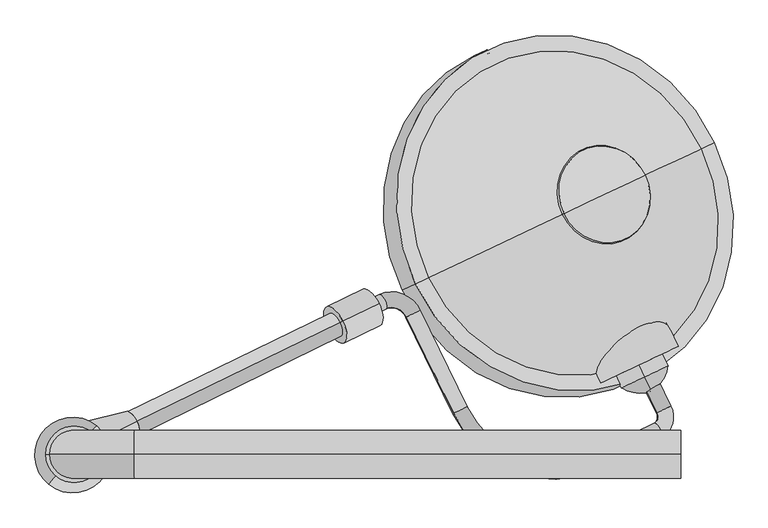
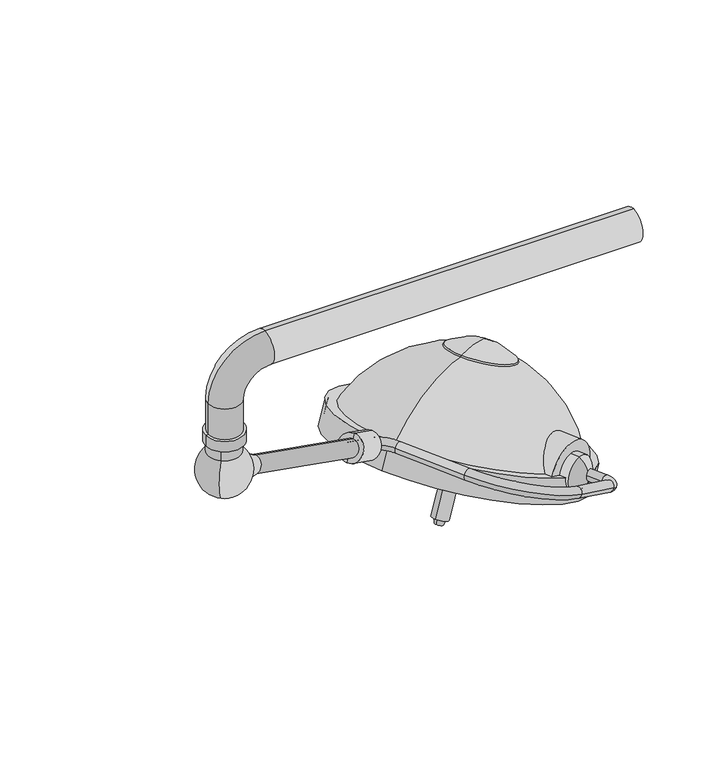
"""IFC4 building model written with IfcOpenShell, lengths in millimetres: proxy geometry, M7485 - Light, Surg, Ceiling Mtd, Dual, Equal Dia Heads : M7485 - Light, Surg, Ceiling Mtd, Dual, Equal Dia Heads."""

from ifc_helpers import new_model, si_unit, point, frame, frame_2d, origin, origin_2d, place, context, project, spatial, polyline, circle_curve, ellipse_curve, trimmed, segment, composite_curve, outline, extrude, source, transform, mapped, element, save
from ifc_brep_helpers import plane_surface, cylinder_surface, revolved_surface, advanced_brep


def specialty_equipment_14047777(model_context):
    return source(origin(), model_context, "Body", "SolidModel", [
        advanced_brep(
        [(-51.3241797, -670.2413617, 1699.7604265), (-72.1798458, -680.4133498, 1710.0915373), (-51.503984, -722.8051486, 1710.0915373), (-30.6483179, -712.6331606, 1699.7604265), (-56.3645035, -739.305827, 1715.2570926), (-45.2298764, -762.1351958, 1715.2570926), (-159.8794514, -789.7934405, 1766.5344952), (-148.7448243, -812.6228093, 1766.5344952), (-351.8212111, -713.8491561, 1828.5211596), (-372.6768772, -724.0211441, 1838.8522704), (-426.0821694, -561.5916279, 1828.5211596), (-446.9378356, -571.7636159, 1838.8522704), (-490.062756, -536.2768664, 1849.1833811), (-478.9281288, -559.1062352, 1849.1833811), (-557.8921303, -597.619552, 1888.2991704), (-569.0267574, -574.7901832, 1888.2991704)],
        [
            (0, 1, circle_curve(frame((-61.7520127, -675.3273558, 1704.9259819), z_axis=(-0.43837114678908723, 0.8987940462991623, 0.0), x_axis=(-0.8210892183528129, -0.40047196991074896, 0.4067366430758003)), 12.7)),
            (1, 0, circle_curve(frame((-61.7520127, -675.3273558, 1704.9259819), z_axis=(-0.43837114678908723, 0.8987940462991623, 0.0), x_axis=(-0.8210892183528129, -0.40047196991074896, 0.4067366430758003)), 12.7)),
            (1, 2),
            (2, 3, circle_curve(frame((-41.0761509, -717.7191546, 1704.9259819), z_axis=(-0.43837114678908723, 0.8987940462991623, 0.0), x_axis=(-0.8210892183528129, -0.40047196991074896, 0.4067366430758003)), 12.7)),
            (3, 0),
            (3, 2, circle_curve(frame((-41.0761509, -717.7191546, 1704.9259819), z_axis=(-0.43837114678908723, 0.8987940462991623, 0.0), x_axis=(-0.8210892183528129, -0.40047196991074896, 0.4067366430758003)), 12.7)),
            (4, 5, circle_curve(frame((-50.79719, -750.7205114, 1715.2570926), z_axis=(0.8210892183528035, 0.4004719699107681, -0.4067366430758003), x_axis=(-0.43837114678910477, 0.8987940462991536, 0.0)), 12.7)),
            (5, 3, circle_curve(frame((-61.9318171, -727.8911427, 1715.2570926), z_axis=(0.36557247320823727, 0.17830160866628114, 0.9135454576426009), x_axis=(0.8210892183528128, 0.400471969910749, -0.4067366430758004)), 38.1)),
            (2, 4, circle_curve(frame((-61.9318171, -727.8911427, 1715.2570926), z_axis=(-0.36557247320823727, -0.17830160866628114, -0.9135454576426009), x_axis=(0.8210892183528128, 0.400471969910749, -0.4067366430758004)), 12.7)),
            (5, 4, circle_curve(frame((-50.79719, -750.7205114, 1715.2570926), z_axis=(0.8210892183528112, 0.4004719699107522, -0.4067366430758003), x_axis=(-0.4383711467890902, 0.8987940462991607, 0.0)), 12.7)),
            (4, 6),
            (6, 7, circle_curve(frame((-154.3121378, -801.2081249, 1766.5344952), z_axis=(0.821089218352813, 0.40047196991074857, -0.40673664307580043), x_axis=(-0.4383711467890869, 0.8987940462991624, 0.0)), 12.7)),
            (7, 5),
            (7, 6, circle_curve(frame((-154.3121378, -801.2081249, 1766.5344952), z_axis=(0.821089218352813, 0.40047196991074857, -0.40673664307580043), x_axis=(-0.4383711467890869, 0.8987940462991624, 0.0)), 12.7)),
            (8, 9, circle_curve(frame((-362.2490441, -718.9351501, 1833.686715), z_axis=(0.4383711467890848, -0.8987940462991635, 0.0), x_axis=(0.8210892183528142, 0.4004719699107463, -0.40673664307580043)), 12.7)),
            (9, 7, circle_curve(frame((-226.6872142, -652.8172279, 1766.5344952), z_axis=(0.36557247320823727, 0.17830160866628114, 0.9135454576426009), x_axis=(0.43837114678909317, -0.8987940462991594, 0.0)), 177.8)),
            (6, 8, circle_curve(frame((-226.6872142, -652.8172279, 1766.5344952), z_axis=(-0.36557247320823727, -0.17830160866628114, -0.9135454576426009), x_axis=(0.43837114678909317, -0.8987940462991594, 0.0)), 152.4)),
            (9, 8, circle_curve(frame((-362.2490441, -718.9351501, 1833.686715), z_axis=(0.4383711467890851, -0.8987940462991633, 0.0), x_axis=(0.821089218352814, 0.40047196991074674, -0.40673664307580043)), 12.7)),
            (8, 10),
            (10, 11, circle_curve(frame((-436.5100025, -566.6776219, 1833.686715), z_axis=(0.43837114678908545, -0.898794046299163, 0.0), x_axis=(0.8210892183528139, 0.400471969910747, -0.4067366430758005)), 12.7)),
            (11, 9),
            (11, 10, circle_curve(frame((-436.5100025, -566.6776219, 1833.686715), z_axis=(0.43837114678908545, -0.898794046299163, 0.0), x_axis=(0.8210892183528139, 0.400471969910747, -0.4067366430758005)), 12.7)),
            (12, 13, circle_curve(frame((-484.4954424, -547.6915508, 1849.1833811), z_axis=(0.8210892183528171, 0.40047196991074047, -0.4067366430758004), x_axis=(-0.4383711467890795, 0.898794046299166, 0.0)), 12.7)),
            (13, 11, circle_curve(frame((-467.7935017, -581.935604, 1849.1833811), z_axis=(-0.36557247320823727, -0.17830160866628114, -0.9135454576426009), x_axis=(0.8210892183528169, 0.4004719699107408, -0.4067366430758004)), 25.4)),
            (10, 12, circle_curve(frame((-467.7935017, -581.935604, 1849.1833811), z_axis=(0.36557247320823727, 0.17830160866628114, 0.9135454576426009), x_axis=(0.8210892183528169, 0.4004719699107408, -0.4067366430758004)), 50.8)),
            (13, 12, circle_curve(frame((-484.4954424, -547.6915508, 1849.1833811), z_axis=(0.8210892183528171, 0.40047196991074047, -0.4067366430758004), x_axis=(-0.4383711467890795, 0.898794046299166, 0.0)), 12.7)),
            (14, 15, circle_curve(frame((-563.4594439, -586.2048676, 1888.2991704), z_axis=(-0.821089218352815, -0.40047196991074563, 0.4067366430757997), x_axis=(-0.438371146789084, 0.8987940462991637, 0.0)), 12.7)),
            (15, 14, circle_curve(frame((-563.4594439, -586.2048676, 1888.2991704), z_axis=(-0.821089218352815, -0.40047196991074563, 0.4067366430757997), x_axis=(-0.438371146789084, 0.8987940462991637, 0.0)), 12.7)),
            (12, 15),
            (14, 13),
        ],
        [
            plane_surface(frame((-671.2712366, -972.6097446, 181.7710423), z_axis=(-0.43837114678908734, 0.8987940462991622, 0.0), x_axis=(0.3655724732082375, 0.17830160866628114, 0.9135454576426008))),
            cylinder_surface(frame((-61.7520127, -675.3273558, 1704.9259819), z_axis=(-0.43837114678908723, 0.8987940462991623, 0.0), x_axis=(-0.8210892183528129, -0.40047196991074896, 0.4067366430758003)), 12.7),
            revolved_surface(trimmed(ellipse_curve(frame((-41.0761509, -717.7191546, 1704.9259819), z_axis=(0.43837114678908723, -0.8987940462991622, 0.0), x_axis=(-0.8210892183528128, -0.4004719699107489, 0.40673664307580043)), 12.7, 12.7), [point((-30.6483179, -712.6331606, 1699.7604265))], [point((-51.503984, -722.8051486, 1710.0915373))], True, "CARTESIAN"), (-671.451041, -1025.1735315, 192.1021531), (0.36557247320823727, 0.17830160866628114, 0.9135454576426009)),
            revolved_surface(trimmed(ellipse_curve(frame((-41.0761509, -717.7191546, 1704.9259819), z_axis=(0.43837114678908723, -0.8987940462991622, 0.0), x_axis=(-0.8210892183528128, -0.4004719699107489, 0.40673664307580043)), 12.7, 12.7), [point((-51.503984, -722.8051486, 1710.0915373))], [point((-30.6483179, -712.6331606, 1699.7604265))], True, "CARTESIAN"), (-671.451041, -1025.1735315, 192.1021531), (0.36557247320823727, 0.17830160866628114, 0.9135454576426009)),
            cylinder_surface(frame((-50.79719, -750.7205114, 1715.2570926), z_axis=(0.821089218352813, 0.40047196991074857, -0.40673664307580043), x_axis=(-0.4383711467890869, 0.8987940462991624, 0.0)), 12.7),
            revolved_surface(trimmed(ellipse_curve(frame((-154.3121378, -801.2081249, 1766.5344952), z_axis=(-0.8210892183528098, -0.40047196991075545, 0.4067366430758005), x_axis=(-0.4383711467890932, 0.8987940462991594, 0.0)), 12.7, 12.7), [point((-148.7448243, -812.6228093, 1766.5344952))], [point((-159.8794514, -789.7934405, 1766.5344952))], True, "CARTESIAN"), (-836.2064381, -950.0996167, 243.3795556), (0.36557247320823727, 0.17830160866628114, 0.9135454576426009)),
            revolved_surface(trimmed(ellipse_curve(frame((-154.3121378, -801.2081249, 1766.5344952), z_axis=(-0.8210892183528098, -0.40047196991075545, 0.4067366430758005), x_axis=(-0.4383711467890932, 0.8987940462991594, 0.0)), 12.7, 12.7), [point((-159.8794514, -789.7934405, 1766.5344952))], [point((-148.7448243, -812.6228093, 1766.5344952))], True, "CARTESIAN"), (-836.2064381, -950.0996167, 243.3795556), (0.36557247320823727, 0.17830160866628114, 0.9135454576426009)),
            cylinder_surface(frame((-362.2490441, -718.9351501, 1833.686715), z_axis=(0.43837114678908556, -0.8987940462991633, 0.0), x_axis=(0.8210892183528139, 0.400471969910747, -0.4067366430758005)), 12.7),
            revolved_surface(trimmed(ellipse_curve(frame((-436.5100025, -566.6776219, 1833.686715), z_axis=(-0.43837114678907957, 0.898794046299166, 0.0), x_axis=(0.821089218352817, 0.4004719699107405, -0.40673664307580043)), 12.7, 12.7), [point((-446.9378356, -571.7636159, 1838.8522704))], [point((-426.0821694, -561.5916279, 1828.5211596))], True, "CARTESIAN"), (-1077.3127256, -879.2179928, 326.0284415), (-0.36557247320823727, -0.17830160866628114, -0.9135454576426009)),
            revolved_surface(trimmed(ellipse_curve(frame((-436.5100025, -566.6776219, 1833.686715), z_axis=(-0.43837114678907957, 0.898794046299166, 0.0), x_axis=(0.821089218352817, 0.4004719699107405, -0.40673664307580043)), 12.7, 12.7), [point((-426.0821694, -561.5916279, 1828.5211596))], [point((-446.9378356, -571.7636159, 1838.8522704))], True, "CARTESIAN"), (-1077.3127256, -879.2179928, 326.0284415), (-0.36557247320823727, -0.17830160866628114, -0.9135454576426009)),
            plane_surface(frame((-1172.9786678, -883.4872565, 365.1442308), z_axis=(-0.821089218352815, -0.40047196991074574, 0.4067366430757996), x_axis=(0.3655724732082366, 0.1783016086662806, 0.9135454576426013))),
            cylinder_surface(frame((-484.4954424, -547.6915508, 1849.1833811), z_axis=(0.8210892183528148, 0.4004719699107455, -0.4067366430757996), x_axis=(-0.438371146789084, 0.8987940462991637, 0.0)), 12.7),
        ],
        [
            (0, [[1, 2]]),
            (1, [[3, 4, 5, -2]]),
            (1, [[-5, 6, -3, -1]]),
            (2, [[7, 8, -4, 9]]),
            (3, [[10, -9, -6, -8]]),
            (4, [[11, 12, 13, -7]]),
            (4, [[-13, 14, -11, -10]]),
            (5, [[15, 16, -12, 17]]),
            (6, [[18, -17, -14, -16]]),
            (7, [[19, 20, 21, -15]]),
            (7, [[-21, 22, -19, -18]]),
            (8, [[23, 24, -20, 25]]),
            (9, [[26, -25, -22, -24]]),
            (10, [[27, 28]]),
            (11, [[29, -27, 30, -23]]),
            (11, [[-30, -28, -29, -26]]),
        ],
    ),
        advanced_brep(
        [(-70.9853036, -666.0888501, 1662.093259), (-79.9012214, -647.2586456, 1662.093259), (-79.9012214, -647.2586456, 1743.3108067), (-70.9853036, -666.0888501, 1743.3108067), (-59.9841849, -689.3229491, 1702.7020328), (-79.9012214, -647.2586456, 1702.7020328)],
        [
            (0, 1),
            (1, 2, circle_curve(frame((-79.9012214, -647.2586456, 1702.7020328), z_axis=(0.4279431442574036, -0.9038056568107367, 0.0), x_axis=(0.0, 0.0, 1.0)), 40.6087738)),
            (2, 3),
            (3, 0, circle_curve(frame((-70.9853036, -666.0888501, 1702.7020328), z_axis=(-0.4279431442574036, 0.9038056568107367, 0.0), x_axis=(0.0, 0.0, 1.0)), 40.6087738)),
            (2, 1, circle_curve(frame((-79.9012214, -647.2586456, 1702.7020328), z_axis=(0.4279431442574036, -0.9038056568107367, 0.0), x_axis=(0.0, 0.0, 1.0)), 40.6087738)),
            (0, 3, circle_curve(frame((-70.9853036, -666.0888501, 1702.7020328), z_axis=(-0.4279431442574036, 0.9038056568107367, 0.0), x_axis=(0.0, 0.0, 1.0)), 40.6087738)),
            (4, 0, circle_curve(frame((-83.4268503, -639.8126019, 1708.9387051), z_axis=(0.9038056568107369, 0.4279431442574031, 0.0), x_axis=(-0.42794314425740326, 0.9038056568107368, 0.0)), 55.1337385)),
            (3, 4, circle_curve(frame((-83.4268503, -639.8126019, 1696.4653606), z_axis=(0.9038056568107367, 0.42794314425740376, 0.0), x_axis=(-0.42794314425740393, 0.9038056568107365, 0.0)), 55.1337385)),
            (1, 5),
            (5, 2),
        ],
        [
            cylinder_surface(frame((-79.9012214, -647.2586456, 1702.7020328), z_axis=(0.4279431442574036, -0.9038056568107367, 0.0), x_axis=(0.0, 0.0, 1.0)), 40.6087738),
            revolved_surface(trimmed(ellipse_curve(frame((-83.4268503, -639.8126019, 1696.4653606), z_axis=(0.9038056568107367, 0.42794314425740376, 0.0), x_axis=(-0.42794314425740393, 0.9038056568107365, 0.0)), 55.1337385, 55.1337385), [point((-70.9853036, -666.0888501, 1743.3108067))], [point((-59.9841849, -689.3229491, 1702.7020328))], True, "CARTESIAN"), (-79.9012214, -647.2586456, 1702.7020328), (0.4279431442574036, -0.9038056568107367, 0.0)),
            revolved_surface(trimmed(ellipse_curve(frame((-83.4268503, -639.8126019, 1696.4653606), z_axis=(0.9038056568107365, 0.42794314425740393, 0.0), x_axis=(-0.4279431442574041, 0.9038056568107364, 0.0)), 55.1337385, 55.1337385), [point((-70.9853036, -666.0888501, 1743.3108067))], [point((-59.9841849, -689.3229491, 1702.7020328))], True, "CARTESIAN"), (-79.9012214, -647.2586456, 1702.7020328), (0.4279431442574036, -0.9038056568107367, 0.0)),
            plane_surface(frame((-79.9012214, -647.2586456, 1702.7020328), z_axis=(-0.42794314425740343, 0.9038056568107368, 0.0), x_axis=(0.0, 0.0, 1.0))),
        ],
        [
            (0, [[1, 2, 3, 4]]),
            (0, [[-3, 5, -1, 6]]),
            (1, [[7, -4, 8]]),
            (2, [[-8, -6, -7]]),
            (3, [[9, 10, -2]]),
            (3, [[-10, -9, -5]]),
        ],
    ),
        advanced_brep(
        [(-198.2891405, -408.2286063, 1882.6946884), (-123.8504881, -372.982632, 1877.268084), (-70.3964825, -347.6726828, 1819.6927814), (-200.9060117, -409.4676693, 1880.0876662), (-70.3964825, -347.6726828, 1815.7966478), (-129.8474904, -375.822154, 1862.3650044)],
        [
            (0, 1, circle_curve(frame((-172.8421817, -396.1797201, 1682.2916913), z_axis=(-0.427943144257401, 0.9038056568107382, 0.0), x_axis=(0.604764027172337, 0.2863498556040709, -0.7431448254773931)), 202.3711557)),
            (1, 2, circle_curve(frame((-222.0261973, -419.4678707, 1706.5205002), z_axis=(-0.42794314425740376, 0.9038056568107369, 0.0), x_axis=(-0.9038056568107369, -0.4279431442574038, 0.0)), 202.3711557)),
            (2, 0, circle_curve(frame((-134.3428115, -377.9506446, 1851.1937349), z_axis=(0.3676108788441171, 0.17406015792255894, 0.9135454576426013), x_axis=(0.8256675523711364, 0.3909455155656434, -0.4067366430757995)), 77.4480344)),
            (0, 2, circle_curve(frame((-134.3428115, -377.9506446, 1851.1937349), z_axis=(0.3676108788441171, 0.17406015792255894, 0.9135454576426013), x_axis=(0.8256675523711364, 0.3909455155656434, -0.4067366430757995)), 77.4480344)),
            (3, 0),
            (2, 4),
            (4, 3, circle_curve(frame((-135.6512471, -378.5701761, 1847.942157), z_axis=(0.3676108788441171, 0.17406015792255894, 0.9135454576426013), x_axis=(0.8256675523711364, 0.3909455155656434, -0.4067366430757995)), 79.0327347)),
            (3, 4, circle_curve(frame((-135.6512471, -378.5701761, 1847.942157), z_axis=(0.3676108788441171, 0.17406015792255894, 0.9135454576426013), x_axis=(0.8256675523711364, 0.3909455155656434, -0.4067366430757995)), 79.0327347)),
            (5, 3, circle_curve(frame((-221.2532479, -419.1018867, 1596.9639329), z_axis=(0.427943144257401, -0.9038056568107382, 0.0), x_axis=(0.604764027172337, 0.2863498556040709, -0.7431448254773931)), 284.0173877)),
            (4, 5, circle_curve(frame((-246.9439851, -431.2661997, 1609.6195886), z_axis=(0.42794314425740376, -0.9038056568107369, 0.0), x_axis=(-0.9038056568107369, -0.4279431442574038, 0.0)), 284.0173877)),
        ],
        [
            revolved_surface(trimmed(ellipse_curve(frame((-222.0261973, -419.4678707, 1706.5205002), z_axis=(-0.42794314425740376, 0.9038056568107369, 0.0), x_axis=(-0.9038056568107369, -0.4279431442574038, 0.0)), 202.3711557, 202.3711557), [point((-123.8504881, -372.982632, 1877.268084))], [point((-70.3964825, -347.6726828, 1819.6927814))], True, "CARTESIAN"), (-169.8512246, -394.7635311, 1762.9521965), (-0.3676108788441171, -0.17406015792255894, -0.9135454576426013)),
            revolved_surface(trimmed(ellipse_curve(frame((-222.0261973, -419.4678707, 1706.5205002), z_axis=(-0.42794314425740376, 0.9038056568107369, 0.0), x_axis=(-0.9038056568107369, -0.42794314425740376, 0.0)), 202.3711557, 202.3711557), [point((-123.8504881, -372.982632, 1877.268084))], [point((-70.3964825, -347.6726828, 1819.6927814))], True, "CARTESIAN"), (-169.8512246, -394.7635311, 1762.9521965), (-0.3676108788441171, -0.17406015792255894, -0.9135454576426013)),
            revolved_surface(polyline([(-70.3964825, -347.6726828, 1819.6927814), (-70.3964825, -347.6726828, 1815.7966478)]), (-169.8512246, -394.7635311, 1762.9521965), (-0.3676108788441171, -0.17406015792255894, -0.9135454576426013)),
            revolved_surface(trimmed(ellipse_curve(frame((-246.9439851, -431.2661997, 1609.6195886), z_axis=(0.42794314425740376, -0.9038056568107369, 0.0), x_axis=(-0.9038056568107369, -0.4279431442574038, 0.0)), 284.0173877, 284.0173877), [point((-70.3964825, -347.6726828, 1815.7966478))], [point((-129.8474904, -375.822154, 1862.3650044))], True, "CARTESIAN"), (-169.8512246, -394.7635311, 1762.9521965), (-0.3676108788441171, -0.17406015792255894, -0.9135454576426013)),
            revolved_surface(trimmed(ellipse_curve(frame((-246.9439851, -431.2661997, 1609.6195886), z_axis=(0.42794314425740376, -0.9038056568107369, 0.0), x_axis=(-0.9038056568107369, -0.42794314425740376, 0.0)), 284.0173877, 284.0173877), [point((-70.3964825, -347.6726828, 1815.7966478))], [point((-129.8474904, -375.822154, 1862.3650044))], True, "CARTESIAN"), (-169.8512246, -394.7635311, 1762.9521965), (-0.3676108788441171, -0.17406015792255894, -0.9135454576426013)),
        ],
        [
            (0, [[1, 2, 3]]),
            (1, [[-2, -1, 4]]),
            (2, [[5, -3, 6, 7]]),
            (2, [[-6, -4, -5, 8]]),
            (3, [[9, -7, 10]]),
            (4, [[-10, -8, -9]]),
        ],
    ),
        advanced_brep(
        [(-266.4821549, -440.5173321, 1522.8158117), (-255.996177, -435.552324, 1517.6502563), (-276.9681328, -445.4823401, 1527.9813671), (-263.0629437, -438.898369, 1507.6425198), (-271.0121339, -442.6622329, 1511.5584142), (-278.9613242, -446.4260968, 1515.4743086)],
        [
            (0, 1),
            (1, 2, circle_curve(frame((-266.4821549, -440.5173321, 1522.8158117), z_axis=(0.36761087884411703, 0.17406015792255897, 0.9135454576426013), x_axis=(-0.8256675523711364, -0.3909455155656434, 0.40673664307579943)), 12.7)),
            (2, 0),
            (2, 1, circle_curve(frame((-266.4821549, -440.5173321, 1522.8158117), z_axis=(0.36761087884411703, 0.17406015792255897, 0.9135454576426013), x_axis=(-0.8256675523711364, -0.3909455155656434, 0.40673664307579943)), 12.7)),
            (3, 4),
            (4, 5),
            (5, 3, circle_curve(frame((-271.0121339, -442.6622329, 1511.5584142), z_axis=(-0.36761087884411703, -0.17406015792255897, -0.9135454576426013), x_axis=(-0.8256675523711364, -0.3909455155656434, 0.40673664307579943)), 9.6275919)),
            (3, 5, circle_curve(frame((-271.0121339, -442.6622329, 1511.5584142), z_axis=(-0.36761087884411703, -0.17406015792255897, -0.9135454576426013), x_axis=(-0.8256675523711364, -0.3909455155656434, 0.40673664307579943)), 9.6275919)),
            (1, 3),
            (5, 2),
        ],
        [
            plane_surface(frame((-266.4821549, -440.5173321, 1522.8158117), z_axis=(0.36761087884411714, 0.1740601579225589, 0.9135454576426014), x_axis=(-0.8256675523711364, -0.3909455155656434, 0.40673664307579943))),
            plane_surface(frame((-271.0121339, -442.6622329, 1511.5584142), z_axis=(-0.36761087884411714, -0.1740601579225589, -0.9135454576426014), x_axis=(-0.8256675523711364, -0.3909455155656434, 0.40673664307579943))),
            revolved_surface(polyline([(-278.9613242, -446.4260968, 1515.4743086), (-276.9681328, -445.4823401, 1527.9813671)]), (-229.1328896, -422.83282, 1615.6320302), (0.36761087884411703, 0.17406015792255897, 0.9135454576426013)),
        ],
        [
            (0, [[1, 2, 3]]),
            (0, [[-3, 4, -1]]),
            (1, [[5, 6, 7]]),
            (1, [[-6, -5, 8]]),
            (2, [[9, -7, 10, -2]]),
            (2, [[-10, -8, -9, -4]]),
        ],
    ),
        advanced_brep(
        [(-229.1328896, -422.83282, 1615.6320302), (-213.4039227, -415.385308, 1607.8836971), (-244.8618565, -430.2803321, 1623.3803632), (-250.753188, -433.06982, 1515.0674786), (-266.4821549, -440.5173321, 1522.8158117), (-282.2111217, -447.9648442, 1530.5641447)],
        [
            (0, 1),
            (1, 2, circle_curve(frame((-229.1328896, -422.83282, 1615.6320302), z_axis=(0.36761087884411703, 0.17406015792255897, 0.9135454576426013), x_axis=(-0.8256675523711364, -0.3909455155656434, 0.40673664307579943)), 19.05)),
            (2, 0),
            (2, 1, circle_curve(frame((-229.1328896, -422.83282, 1615.6320302), z_axis=(0.36761087884411703, 0.17406015792255897, 0.9135454576426013), x_axis=(-0.8256675523711364, -0.3909455155656434, 0.40673664307579943)), 19.05)),
            (3, 4),
            (4, 5),
            (5, 3, circle_curve(frame((-266.4821549, -440.5173321, 1522.8158117), z_axis=(-0.36761087884411703, -0.17406015792255897, -0.9135454576426013), x_axis=(-0.8256675523711364, -0.3909455155656434, 0.40673664307579943)), 19.05)),
            (3, 5, circle_curve(frame((-266.4821549, -440.5173321, 1522.8158117), z_axis=(-0.36761087884411703, -0.17406015792255897, -0.9135454576426013), x_axis=(-0.8256675523711364, -0.3909455155656434, 0.40673664307579943)), 19.05)),
            (1, 3),
            (5, 2),
        ],
        [
            plane_surface(frame((-229.1328896, -422.83282, 1615.6320302), z_axis=(0.36761087884411714, 0.1740601579225589, 0.9135454576426014), x_axis=(-0.8256675523711364, -0.3909455155656434, 0.40673664307579943))),
            plane_surface(frame((-266.4821549, -440.5173321, 1522.8158117), z_axis=(-0.36761087884411714, -0.1740601579225589, -0.9135454576426014), x_axis=(-0.8256675523711364, -0.3909455155656434, 0.40673664307579943))),
            cylinder_surface(frame((-229.1328896, -422.83282, 1615.6320302), z_axis=(0.36761087884411703, 0.17406015792255897, 0.9135454576426013), x_axis=(-0.8256675523711364, -0.3909455155656434, 0.40673664307579943)), 19.05),
        ],
        [
            (0, [[1, 2, 3]]),
            (0, [[-3, 4, -1]]),
            (1, [[5, 6, 7]]),
            (1, [[-6, -5, 8]]),
            (2, [[9, -7, 10, -2]]),
            (2, [[-10, -8, -9, -4]]),
        ],
    ),
        advanced_brep(
        [(-222.1299023, -419.516974, 1633.0350712), (-185.4289796, -402.1394459, 1614.9556274), (-258.830825, -436.8945022, 1651.1145149), (-192.4319669, -405.4552919, 1597.5525864), (-229.1328896, -422.83282, 1615.6320302), (-265.8338123, -440.2103482, 1633.711474)],
        [
            (0, 1),
            (1, 2, circle_curve(frame((-222.1299023, -419.516974, 1633.0350712), z_axis=(0.3676108788441165, 0.1740601579225587, 0.9135454576426016), x_axis=(-0.8256675523711366, -0.3909455155656435, 0.4067366430757988)), 44.45)),
            (2, 0),
            (2, 1, circle_curve(frame((-222.1299023, -419.516974, 1633.0350712), z_axis=(0.3676108788441165, 0.1740601579225587, 0.9135454576426016), x_axis=(-0.8256675523711366, -0.3909455155656435, 0.4067366430757988)), 44.45)),
            (3, 4),
            (4, 5),
            (5, 3, circle_curve(frame((-229.1328896, -422.83282, 1615.6320302), z_axis=(-0.3676108788441165, -0.1740601579225587, -0.9135454576426016), x_axis=(-0.8256675523711366, -0.3909455155656435, 0.4067366430757988)), 44.45)),
            (3, 5, circle_curve(frame((-229.1328896, -422.83282, 1615.6320302), z_axis=(-0.3676108788441165, -0.1740601579225587, -0.9135454576426016), x_axis=(-0.8256675523711366, -0.3909455155656435, 0.4067366430757988)), 44.45)),
            (1, 3),
            (5, 2),
        ],
        [
            plane_surface(frame((-222.1299023, -419.516974, 1633.0350712), z_axis=(0.3676108788441166, 0.17406015792255863, 0.9135454576426016), x_axis=(-0.8256675523711366, -0.3909455155656435, 0.4067366430757988))),
            plane_surface(frame((-229.1328896, -422.83282, 1615.6320302), z_axis=(-0.3676108788441166, -0.17406015792255863, -0.9135454576426016), x_axis=(-0.8256675523711366, -0.3909455155656435, 0.4067366430757988))),
            cylinder_surface(frame((-222.1299023, -419.516974, 1633.0350712), z_axis=(0.3676108788441165, 0.1740601579225587, 0.9135454576426016), x_axis=(-0.8256675523711366, -0.3909455155656435, 0.4067366430757988)), 44.45),
        ],
        [
            (0, [[1, 2, 3]]),
            (0, [[-3, 4, -1]]),
            (1, [[5, 6, 7]]),
            (1, [[-6, -5, 8]]),
            (2, [[9, -7, 10, -2]]),
            (2, [[-10, -8, -9, -4]]),
        ],
    ),
        advanced_brep(
        [(-217.8648709, -417.4975233, 1643.6340505), (-170.6779703, -395.1549871, 1620.3890514), (-265.0517715, -439.8400595, 1666.8790497), (-179.2080332, -399.1938885, 1611.8910927), (-222.1299023, -419.516974, 1633.0350712), (-265.0517715, -439.8400595, 1654.1790497)],
        [
            (0, 1),
            (1, 2, circle_curve(frame((-217.8648709, -417.4975233, 1643.6340505), z_axis=(0.36761087884411725, 0.17406015792255908, 0.9135454576426012), x_axis=(-0.8256675523711363, -0.39094551556564333, 0.4067366430757997)), 57.15)),
            (2, 0),
            (2, 1, circle_curve(frame((-217.8648709, -417.4975233, 1643.6340505), z_axis=(0.36761087884411725, 0.17406015792255908, 0.9135454576426012), x_axis=(-0.8256675523711363, -0.39094551556564333, 0.4067366430757997)), 57.15)),
            (3, 4),
            (4, 5),
            (5, 3, circle_curve(frame((-222.1299023, -419.516974, 1633.0350712), z_axis=(-0.36761087884411725, -0.17406015792255908, -0.9135454576426012), x_axis=(-0.8256675523711363, -0.39094551556564333, 0.4067366430757997)), 51.9844446)),
            (3, 5, circle_curve(frame((-222.1299023, -419.516974, 1633.0350712), z_axis=(-0.36761087884411725, -0.17406015792255908, -0.9135454576426012), x_axis=(-0.8256675523711363, -0.39094551556564333, 0.4067366430757997)), 51.9844446)),
            (1, 3),
            (5, 2),
        ],
        [
            plane_surface(frame((-217.8648709, -417.4975233, 1643.6340505), z_axis=(0.36761087884411736, 0.17406015792255902, 0.9135454576426013), x_axis=(-0.8256675523711363, -0.39094551556564333, 0.4067366430757997))),
            plane_surface(frame((-222.1299023, -419.516974, 1633.0350712), z_axis=(-0.36761087884411736, -0.17406015792255902, -0.9135454576426013), x_axis=(-0.8256675523711363, -0.39094551556564333, 0.4067366430757997))),
            revolved_surface(polyline([(-265.0517715, -439.8400595, 1654.1790497), (-265.0517715, -439.8400595, 1666.8790497)]), (-217.8648709, -417.4975233, 1643.6340505), (0.36761087884411725, 0.17406015792255908, 0.9135454576426012)),
        ],
        [
            (0, [[1, 2, 3]]),
            (0, [[-3, 4, -1]]),
            (1, [[5, 6, 7]]),
            (1, [[-6, -5, 8]]),
            (2, [[9, -7, 10, -2]]),
            (2, [[-10, -8, -9, -4]]),
        ],
    ),
        extrude(outline(composite_curve([segment(polyline([(25.1937137, 4.6953207), (-31.6273953, 132.3176211)]), True, "CONTINUOUS"), segment(trimmed(circle_curve(frame_2d((0.0, 69.9387006)), 69.9387006), [point((-31.6273953, 132.3176211))], [point((25.1937137, 4.6953207))], False, "CARTESIAN"), True, "CONTINUOUS")], self_intersect=False)), frame((-144.6400085, -677.9118285, 1699.0600142), z_axis=(-0.42794314425740343, 0.9038056568107368, 0.0), x_axis=(0.0, 0.0, 1.0)), (0.0, 0.0, 1.0), 84.2600986),
        advanced_brep(
        [(-411.8184564, -509.3326503, 1801.7370584), (-129.8408016, -375.8189869, 1862.3816266), (18.1066381, -305.7673203, 1589.9492884), (-406.0906916, -506.6206096, 1798.9154726), (12.3788733, -308.479361, 1592.7708742), (-132.17953, -376.9263519, 1856.5696802)],
        [
            (0, 1, circle_curve(frame((-226.1466857, -421.4188817, 1577.7194701), z_axis=(-0.42794314425740104, 0.9038056568107381, 0.0), x_axis=(0.6047640271723369, 0.28634985560407084, -0.7431448254773931)), 303.9518334)),
            (1, 2, circle_curve(frame((-256.5953432, -435.8360234, 1592.718951), z_axis=(-0.4279431442574038, 0.9038056568107369, 0.0), x_axis=(-0.9038056568107368, -0.4279431442574038, 0.0)), 303.9518334)),
            (2, 0, circle_curve(frame((-196.8559092, -407.5499853, 1695.8431734), z_axis=(0.3676108788441172, 0.17406015792255902, 0.9135454576426013), x_axis=(0.8256675523711364, 0.3909455155656434, -0.4067366430757996)), 260.35)),
            (0, 2, circle_curve(frame((-196.8559092, -407.5499853, 1695.8431734), z_axis=(0.3676108788441172, 0.17406015792255902, 0.9135454576426013), x_axis=(0.8256675523711364, 0.3909455155656434, -0.4067366430757996)), 260.35)),
            (3, 0),
            (2, 4),
            (4, 3, circle_curve(frame((-196.8559092, -407.5499853, 1695.8431734), z_axis=(0.3676108788441172, 0.17406015792255902, 0.9135454576426013), x_axis=(0.8256675523711364, 0.3909455155656434, -0.4067366430757996)), 253.412868)),
            (3, 4, circle_curve(frame((-196.8559092, -407.5499853, 1695.8431734), z_axis=(0.3676108788441172, 0.17406015792255902, 0.9135454576426013), x_axis=(0.8256675523711364, 0.3909455155656434, -0.4067366430757996)), 253.412868)),
            (5, 3, circle_curve(frame((-226.1466857, -421.4188817, 1577.7194701), z_axis=(0.42794314425740104, -0.9038056568107381, 0.0), x_axis=(0.6047640271723369, 0.28634985560407084, -0.7431448254773931)), 297.6018334)),
            (4, 5, circle_curve(frame((-256.5953432, -435.8360234, 1592.718951), z_axis=(0.4279431442574038, -0.9038056568107369, 0.0), x_axis=(-0.9038056568107368, -0.4279431442574038, 0.0)), 297.6018334)),
        ],
        [
            revolved_surface(trimmed(ellipse_curve(frame((-256.5953432, -435.8360234, 1592.718951), z_axis=(-0.4279431442574038, 0.9038056568107369, 0.0), x_axis=(-0.9038056568107368, -0.4279431442574038, 0.0)), 303.9518334, 303.9518334), [point((-129.8408016, -375.8189869, 1862.3816266))], [point((18.1066381, -305.7673203, 1589.9492884))], True, "CARTESIAN"), (-196.8559092, -407.5499853, 1695.8431734), (-0.3676108788441172, -0.17406015792255902, -0.9135454576426013)),
            revolved_surface(trimmed(ellipse_curve(frame((-256.5953432, -435.8360234, 1592.718951), z_axis=(-0.4279431442574037, 0.9038056568107367, 0.0), x_axis=(-0.9038056568107368, -0.42794314425740376, 0.0)), 303.9518334, 303.9518334), [point((-129.8408016, -375.8189869, 1862.3816266))], [point((18.1066381, -305.7673203, 1589.9492884))], True, "CARTESIAN"), (-196.8559092, -407.5499853, 1695.8431734), (-0.3676108788441172, -0.17406015792255902, -0.9135454576426013)),
            plane_surface(frame((-196.8559092, -407.5499853, 1695.8431734), z_axis=(-0.3676108788441172, -0.17406015792255894, -0.9135454576426013), x_axis=(0.8256675523711363, 0.39094551556564333, -0.40673664307579954))),
            revolved_surface(trimmed(ellipse_curve(frame((-256.5953432, -435.8360234, 1592.718951), z_axis=(0.4279431442574038, -0.9038056568107369, 0.0), x_axis=(-0.9038056568107368, -0.4279431442574038, 0.0)), 297.6018334, 297.6018334), [point((12.3788733, -308.479361, 1592.7708742))], [point((-132.17953, -376.9263519, 1856.5696802))], True, "CARTESIAN"), (-196.8559092, -407.5499853, 1695.8431734), (-0.3676108788441172, -0.17406015792255902, -0.9135454576426013)),
            revolved_surface(trimmed(ellipse_curve(frame((-256.5953432, -435.8360234, 1592.718951), z_axis=(0.4279431442574037, -0.9038056568107367, 0.0), x_axis=(-0.9038056568107368, -0.42794314425740376, 0.0)), 297.6018334, 297.6018334), [point((12.3788733, -308.479361, 1592.7708742))], [point((-132.17953, -376.9263519, 1856.5696802))], True, "CARTESIAN"), (-196.8559092, -407.5499853, 1695.8431734), (-0.3676108788441172, -0.17406015792255902, -0.9135454576426013)),
        ],
        [
            (0, [[1, 2, 3]]),
            (1, [[-2, -1, 4]]),
            (2, [[5, -3, 6, 7]]),
            (2, [[-6, -4, -5, 8]]),
            (3, [[9, -7, 10]]),
            (4, [[-10, -8, -9]]),
        ],
    ),
        advanced_brep(
        [(-453.799374, -529.2102044, 1759.8590463), (-432.7904123, -519.2626664, 1812.0681692), (39.0785939, -295.8373042, 1579.6181777), (18.0696322, -305.7848423, 1527.4090547), (-448.556385, -526.7277004, 1757.2762686), (12.8266432, -308.2673463, 1529.9918324), (-429.8817524, -517.8854444, 1803.6843778), (31.5012759, -299.4250903, 1576.3999417), (-199.1902382, -408.6552673, 1690.0421598), (-196.8559092, -407.5499853, 1695.8431734)],
        [
            (0, 1),
            (1, 2, circle_curve(frame((-196.8559092, -407.5499853, 1695.8431734), z_axis=(-0.3676108788441169, -0.17406015792255886, -0.9135454576426014), x_axis=(0.8256675523711365, 0.39094551556564344, -0.40673664307579926)), 285.75)),
            (2, 3),
            (3, 0, circle_curve(frame((-217.8648709, -417.4975233, 1643.6340505), z_axis=(0.3676108788441169, 0.17406015792255886, 0.9135454576426014), x_axis=(0.8256675523711365, 0.39094551556564344, -0.40673664307579926)), 285.75)),
            (2, 1, circle_curve(frame((-196.8559092, -407.5499853, 1695.8431734), z_axis=(-0.3676108788441169, -0.17406015792255886, -0.9135454576426014), x_axis=(0.8256675523711365, 0.39094551556564344, -0.40673664307579926)), 285.75)),
            (0, 3, circle_curve(frame((-217.8648709, -417.4975233, 1643.6340505), z_axis=(0.3676108788441169, 0.17406015792255886, 0.9135454576426014), x_axis=(0.8256675523711365, 0.39094551556564344, -0.40673664307579926)), 285.75)),
            (4, 0),
            (3, 5),
            (5, 4, circle_curve(frame((-217.8648709, -417.4975233, 1643.6340505), z_axis=(0.3676108788441169, 0.17406015792255886, 0.9135454576426014), x_axis=(0.8256675523711365, 0.39094551556564344, -0.40673664307579926)), 279.4)),
            (4, 5, circle_curve(frame((-217.8648709, -417.4975233, 1643.6340505), z_axis=(0.3676108788441169, 0.17406015792255886, 0.9135454576426014), x_axis=(0.8256675523711365, 0.39094551556564344, -0.40673664307579926)), 279.4)),
            (6, 4),
            (5, 7),
            (7, 6, circle_curve(frame((-199.1902382, -408.6552673, 1690.0421598), z_axis=(0.3676108788441169, 0.17406015792255886, 0.9135454576426014), x_axis=(0.8256675523711365, 0.39094551556564344, -0.40673664307579926)), 279.4)),
            (6, 7, circle_curve(frame((-199.1902382, -408.6552673, 1690.0421598), z_axis=(0.3676108788441169, 0.17406015792255886, 0.9135454576426014), x_axis=(0.8256675523711365, 0.39094551556564344, -0.40673664307579926)), 279.4)),
            (8, 6),
            (7, 8),
            (1, 9),
            (9, 2),
        ],
        [
            cylinder_surface(frame((-217.8648709, -417.4975233, 1643.6340505), z_axis=(-0.3676108788441169, -0.17406015792255886, -0.9135454576426014), x_axis=(0.8256675523711365, 0.39094551556564344, -0.40673664307579926)), 285.75),
            plane_surface(frame((-217.8648709, -417.4975233, 1643.6340505), z_axis=(-0.3676108788441169, -0.1740601579225588, -0.9135454576426014), x_axis=(0.8256675523711364, 0.3909455155656434, -0.4067366430757992))),
            revolved_surface(polyline([(12.826643216697537, -308.26734625843943, 1529.9918323853624), (31.50127590111487, -299.42509021744286, 1576.3999417308635)]), (-217.8648709, -417.4975233, 1643.6340505), (-0.3676108788441169, -0.17406015792255886, -0.9135454576426014)),
            plane_surface(frame((-199.1902382, -408.6552673, 1690.0421598), z_axis=(-0.3676108788441169, -0.1740601579225588, -0.9135454576426014), x_axis=(0.8256675523711364, 0.3909455155656434, -0.4067366430757992))),
            plane_surface(frame((-196.8559092, -407.5499853, 1695.8431734), z_axis=(0.3676108788441169, 0.1740601579225588, 0.9135454576426014), x_axis=(0.8256675523711364, 0.3909455155656434, -0.4067366430757992))),
        ],
        [
            (0, [[1, 2, 3, 4]]),
            (0, [[-3, 5, -1, 6]]),
            (1, [[7, -4, 8, 9]]),
            (1, [[-8, -6, -7, 10]]),
            (2, [[11, -9, 12, 13]]),
            (2, [[-12, -10, -11, 14]]),
            (3, [[15, -13, 16]]),
            (3, [[-16, -14, -15]]),
            (4, [[17, 18, -2]]),
            (4, [[-18, -17, -5]]),
        ],
    ),
        advanced_brep(
        [(-571.2157425, -589.9878672, 1857.3919398), (-559.1556073, -584.1057463, 1886.167212), (-547.0954721, -578.2236253, 1914.9424843), (-514.3170471, -562.2365192, 1827.8720542), (-490.1967767, -550.4722773, 1885.4225987), (-502.2569119, -556.3543983, 1856.6473264)],
        [
            (0, 1),
            (1, 2),
            (2, 0, circle_curve(frame((-559.1556073, -584.1057463, 1886.167212), z_axis=(-0.8145840431031117, -0.3972991839471335, 0.42261826174069883), x_axis=(0.37984677750984175, 0.18526365205327952, 0.9063077870366504)), 31.75)),
            (0, 2, circle_curve(frame((-559.1556073, -584.1057463, 1886.167212), z_axis=(-0.8145840431031117, -0.3972991839471335, 0.42261826174069883), x_axis=(0.37984677750984175, 0.18526365205327952, 0.9063077870366504)), 31.75)),
            (3, 0),
            (2, 4),
            (4, 3, circle_curve(frame((-502.2569119, -556.3543983, 1856.6473264), z_axis=(-0.8145840431031117, -0.3972991839471335, 0.42261826174069883), x_axis=(0.37984677750984175, 0.18526365205327952, 0.9063077870366504)), 31.75)),
            (3, 4, circle_curve(frame((-502.2569119, -556.3543983, 1856.6473264), z_axis=(-0.8145840431031117, -0.3972991839471335, 0.42261826174069883), x_axis=(0.37984677750984175, 0.18526365205327952, 0.9063077870366504)), 31.75)),
            (5, 3),
            (4, 5),
        ],
        [
            plane_surface(frame((-559.1556073, -584.1057463, 1886.167212), z_axis=(-0.8145840431031117, -0.3972991839471334, 0.42261826174069883), x_axis=(0.37984677750984175, 0.18526365205327952, 0.9063077870366504))),
            cylinder_surface(frame((-559.1556073, -584.1057463, 1886.167212), z_axis=(0.8145840431031117, 0.3972991839471335, -0.42261826174069883), x_axis=(0.37984677750984175, 0.18526365205327952, 0.9063077870366504)), 31.75),
            plane_surface(frame((-502.2569119, -556.3543983, 1856.6473264), z_axis=(0.8145840431031117, 0.3972991839471334, -0.42261826174069883), x_axis=(0.37984677750984175, 0.18526365205327952, 0.9063077870366504))),
        ],
        [
            (0, [[1, 2, 3]]),
            (0, [[-2, -1, 4]]),
            (1, [[5, -3, 6, 7]]),
            (1, [[-6, -4, -5, 8]]),
            (2, [[9, -7, 10]]),
            (2, [[-10, -8, -9]]),
        ],
    ),
        extrude(outline(composite_curve([segment(trimmed(circle_curve(origin_2d(), 20.2288163), [point((0.0, 20.2288164))], [point((0.0, -20.2288163))], False, "CARTESIAN"), True, "CONTINUOUS"), segment(trimmed(circle_curve(origin_2d(), 20.2288163), [point((0.0, -20.2288163))], [point((0.0, 20.2288164))], False, "CARTESIAN"), True, "CONTINUOUS")], self_intersect=False)), frame((-559.1556073, -584.1057463, 1886.167212), z_axis=(-0.8145840431031119, -0.39729918394713354, 0.4226182617406987), x_axis=(0.4383711467890842, -0.8987940462991637, 0.0)), (0.0, 0.0, 1.0), 393.7),
        advanced_brep(
        [(-940.9549717, -770.3217386, 2081.4066897), (-928.0978809, -764.0509164, 2115.1067436), (-953.8120625, -776.5925608, 2047.7066358), (-872.3231351, -736.8477552, 2072.3001347), (-879.8573451, -740.522435, 2052.5520217), (-887.391555, -744.1971147, 2032.8039086)],
        [
            (0, 1),
            (1, 2, circle_curve(frame((-940.9549717, -770.3217386, 2081.4066897), z_axis=(-0.8273442818725376, -0.40352276823286415, 0.39073112848927416), x_axis=(-0.3511868119899131, -0.1712852528820361, -0.9205048534524402)), 36.6104033)),
            (2, 0),
            (2, 1, circle_curve(frame((-940.9549717, -770.3217386, 2081.4066897), z_axis=(-0.8273442818725376, -0.40352276823286415, 0.39073112848927416), x_axis=(-0.3511868119899131, -0.1712852528820361, -0.9205048534524402)), 36.6104033)),
            (3, 4),
            (4, 5),
            (5, 3, circle_curve(frame((-879.8573451, -740.522435, 2052.5520217), z_axis=(0.8273442818725376, 0.40352276823286415, -0.39073112848927416), x_axis=(-0.3511868119899131, -0.1712852528820361, -0.9205048534524402)), 21.4535676)),
            (3, 5, circle_curve(frame((-879.8573451, -740.522435, 2052.5520217), z_axis=(0.8273442818725376, 0.40352276823286415, -0.39073112848927416), x_axis=(-0.3511868119899131, -0.1712852528820361, -0.9205048534524402)), 21.4535676)),
            (1, 3),
            (5, 2),
        ],
        [
            plane_surface(frame((-940.9549717, -770.3217386, 2081.4066897), z_axis=(-0.8273442818725375, -0.40352276823286404, 0.39073112848927416), x_axis=(-0.35118681198991314, -0.17128525288203614, -0.9205048534524403))),
            plane_surface(frame((-879.8573451, -740.522435, 2052.5520217), z_axis=(0.8273442818725375, 0.40352276823286404, -0.39073112848927416), x_axis=(-0.35118681198991314, -0.17128525288203614, -0.9205048534524403))),
            revolved_surface(polyline([(-887.391555, -744.1971147, 2032.8039086), (-953.8120625, -776.5925608, 2047.7066358)]), (-921.8864346, -761.0213916, 2072.401163), (-0.8273442818725374, -0.40352276823286404, 0.39073112848927405)),
        ],
        [
            (0, [[1, 2, 3]]),
            (0, [[-3, 4, -1]]),
            (1, [[5, 6, 7]]),
            (1, [[-6, -5, 8]]),
            (2, [[9, -7, 10, -2]]),
            (2, [[-10, -8, -9, -4]]),
        ],
    ),
        advanced_brep(
        [(-973.5341458, -789.78967, 2175.962195), (-997.5112527, -819.3989311, 2175.962195), (-949.5570389, -760.1804089, 2175.962195), (-997.5112527, -819.3989311, 2150.1869575), (-973.5341458, -789.78967, 2044.1286543), (-949.5570389, -760.1804089, 2150.1869575)],
        [
            (0, 1),
            (1, 2, circle_curve(frame((-973.5341458, -789.78967, 2175.962195), z_axis=(0.0, 0.0, 1.0), x_axis=(0.62932039104983, 0.7771459614569771, 0.0)), 38.1)),
            (2, 0),
            (2, 1, circle_curve(frame((-973.5341458, -789.78967, 2175.962195), z_axis=(0.0, 0.0, 1.0), x_axis=(0.62932039104983, 0.7771459614569771, 0.0)), 38.1)),
            (3, 4, circle_curve(frame((-973.5341458, -789.78967, 2104.0012588), z_axis=(0.7771459614569792, -0.6293203910498274, 0.0), x_axis=(-0.6293203910498274, -0.7771459614569792, 0.0)), 59.8726045)),
            (4, 5, circle_curve(frame((-973.5341458, -789.78967, 2104.0012588), z_axis=(0.7771459614569772, -0.6293203910498298, 0.0), x_axis=(0.6293203910498298, 0.7771459614569772, 0.0)), 59.8726045)),
            (5, 3, circle_curve(frame((-973.5341458, -789.78967, 2150.1869575), z_axis=(0.0, 0.0, -1.0), x_axis=(0.62932039104983, 0.7771459614569771, 0.0)), 38.1)),
            (3, 5, circle_curve(frame((-973.5341458, -789.78967, 2150.1869575), z_axis=(0.0, 0.0, -1.0), x_axis=(0.62932039104983, 0.7771459614569771, 0.0)), 38.1)),
            (1, 3),
            (5, 2),
        ],
        [
            plane_surface(frame((-973.5341458, -789.78967, 2175.962195), z_axis=(0.0, 0.0, 1.0000000000000002), x_axis=(0.62932039104983, 0.7771459614569771, 0.0))),
            revolved_surface(trimmed(ellipse_curve(frame((-973.5341458, -789.78967, 2104.0012588), z_axis=(0.7771459614569772, -0.6293203910498298, 0.0), x_axis=(0.6293203910498298, 0.7771459614569772, 0.0)), 59.8726045, 59.8726045), [point((-973.5341458, -789.78967, 2044.1286543))], [point((-949.5570389, -760.1804089, 2150.1869575))], True, "CARTESIAN"), (-973.5341458, -789.78967, 2175.962195), (0.0, 0.0, 1.0)),
            cylinder_surface(frame((-973.5341458, -789.78967, 2175.962195), z_axis=(0.0, 0.0, 1.0), x_axis=(0.62932039104983, 0.7771459614569771, 0.0)), 38.1),
        ],
        [
            (0, [[1, 2, 3]]),
            (0, [[-3, 4, -1]]),
            (1, [[5, 6, 7]]),
            (1, [[-6, -5, 8]]),
            (2, [[9, -7, 10, -2]]),
            (2, [[-10, -8, -9, -4]]),
        ],
    ),
        advanced_brep(
        [(-927.1, -788.5674111, 2175.962195), (-971.55, -788.5674111, 2175.962195), (-1016.0, -788.5674111, 2175.962195), (-927.1, -788.5674111, 2201.362195), (-1016.0, -788.5674111, 2201.362195), (-971.55, -788.5674111, 2201.362195)],
        [
            (0, 1),
            (1, 2),
            (2, 0, circle_curve(frame((-971.55, -788.5674111, 2175.962195), z_axis=(0.0, 0.0, -1.0), x_axis=(-1.0, 0.0, 0.0)), 44.45)),
            (0, 2, circle_curve(frame((-971.55, -788.5674111, 2175.962195), z_axis=(0.0, 0.0, -1.0), x_axis=(-1.0, 0.0, 0.0)), 44.45)),
            (3, 0),
            (2, 4),
            (4, 3, circle_curve(frame((-971.55, -788.5674111, 2201.362195), z_axis=(0.0, 0.0, -1.0), x_axis=(-1.0, 0.0, 0.0)), 44.45)),
            (3, 4, circle_curve(frame((-971.55, -788.5674111, 2201.362195), z_axis=(0.0, 0.0, -1.0), x_axis=(-1.0, 0.0, 0.0)), 44.45)),
            (5, 3),
            (4, 5),
        ],
        [
            plane_surface(frame((-971.55, -788.5674111, 2175.962195), z_axis=(0.0, 0.0, -1.0), x_axis=(-1.0, 0.0, 0.0))),
            cylinder_surface(frame((-971.55, -788.5674111, 2201.362195), z_axis=(0.0, 0.0, 1.0), x_axis=(-1.0, 0.0, 0.0)), 44.45),
            plane_surface(frame((-971.55, -788.5674111, 2201.362195), z_axis=(0.0, 0.0, 1.0), x_axis=(-1.0, 0.0, 0.0))),
        ],
        [
            (0, [[1, 2, 3]]),
            (0, [[-2, -1, 4]]),
            (1, [[5, -3, 6, 7]]),
            (1, [[-6, -4, -5, 8]]),
            (2, [[9, -7, 10]]),
            (2, [[-10, -8, -9]]),
        ],
    ),
        advanced_brep(
        [(-14.4818275, -788.5674111, 2334.712195), (-14.4818275, -788.5674111, 2410.912195), (-876.3, -788.5674111, 2410.912195), (-876.3, -788.5674111, 2334.712195), (-1009.65, -788.5674111, 2277.562195), (-933.45, -788.5674111, 2277.562195), (-933.45, -788.5674111, 2201.362195), (-1009.65, -788.5674111, 2201.362195)],
        [
            (0, 1, circle_curve(frame((-14.4818275, -788.5674111, 2372.812195), z_axis=(1.0, 0.0, 0.0), x_axis=(0.0, 0.0, 1.0)), 38.1)),
            (1, 0, circle_curve(frame((-14.4818275, -788.5674111, 2372.812195), z_axis=(1.0, 0.0, 0.0), x_axis=(0.0, 0.0, 1.0)), 38.1)),
            (1, 2),
            (2, 3, circle_curve(frame((-876.3, -788.5674111, 2372.812195), z_axis=(1.0, 0.0, 0.0), x_axis=(0.0, 0.0, 1.0)), 38.1)),
            (3, 0),
            (3, 2, circle_curve(frame((-876.3, -788.5674111, 2372.812195), z_axis=(1.0, 0.0, 0.0), x_axis=(0.0, 0.0, 1.0)), 38.1)),
            (4, 5, circle_curve(frame((-971.55, -788.5674111, 2277.562195), z_axis=(0.0, 0.0, 1.0), x_axis=(-1.0, 0.0, 0.0)), 38.1)),
            (5, 3, circle_curve(frame((-876.3, -788.5674111, 2277.562195), z_axis=(0.0, 1.0, 0.0), x_axis=(0.0, 0.0, 1.0)), 57.15)),
            (2, 4, circle_curve(frame((-876.3, -788.5674111, 2277.562195), z_axis=(0.0, -1.0, 0.0), x_axis=(0.0, 0.0, 1.0)), 133.35)),
            (5, 4, circle_curve(frame((-971.55, -788.5674111, 2277.562195), z_axis=(0.0, 0.0, 1.0), x_axis=(-1.0, 0.0, 0.0)), 38.1)),
            (6, 7, circle_curve(frame((-971.55, -788.5674111, 2201.362195), z_axis=(0.0, 0.0, -1.0), x_axis=(-1.0, 0.0, 0.0)), 38.1)),
            (7, 6, circle_curve(frame((-971.55, -788.5674111, 2201.362195), z_axis=(0.0, 0.0, -1.0), x_axis=(-1.0, 0.0, 0.0)), 38.1)),
            (4, 7),
            (6, 5),
        ],
        [
            plane_surface(frame((-14.4818275, -788.5674111, 2372.812195), z_axis=(1.0, 0.0, 0.0), x_axis=(0.0, -1.0, 0.0))),
            cylinder_surface(frame((-14.4818275, -788.5674111, 2372.812195), z_axis=(1.0, 0.0, 0.0), x_axis=(0.0, 0.0, 1.0)), 38.1),
            revolved_surface(trimmed(ellipse_curve(frame((-876.3, -788.5674111, 2372.812195), z_axis=(-1.0, 0.0, 0.0), x_axis=(0.0, 0.0, 1.0)), 38.1, 38.1), [point((-876.3, -788.5674111, 2334.712195))], [point((-876.3, -788.5674111, 2410.912195))], True, "CARTESIAN"), (-876.3, -788.5674111, 2277.562195), (0.0, 1.0, 0.0)),
            revolved_surface(trimmed(ellipse_curve(frame((-876.3, -788.5674111, 2372.812195), z_axis=(-1.0, 0.0, 0.0), x_axis=(0.0, 0.0, 1.0)), 38.1, 38.1), [point((-876.3, -788.5674111, 2410.912195))], [point((-876.3, -788.5674111, 2334.712195))], True, "CARTESIAN"), (-876.3, -788.5674111, 2277.562195), (0.0, 1.0, 0.0)),
            plane_surface(frame((-971.55, -788.5674111, 2201.362195), z_axis=(0.0, 0.0, -1.0), x_axis=(0.0, -1.0, 0.0))),
            cylinder_surface(frame((-971.55, -788.5674111, 2277.562195), z_axis=(0.0, 0.0, 1.0), x_axis=(-1.0, 0.0, 0.0)), 38.1),
        ],
        [
            (0, [[1, 2]]),
            (1, [[3, 4, 5, -2]]),
            (1, [[-5, 6, -3, -1]]),
            (2, [[7, 8, -4, 9]]),
            (3, [[10, -9, -6, -8]]),
            (4, [[11, 12]]),
            (5, [[13, -11, 14, -7]]),
            (5, [[-14, -12, -13, -10]]),
        ],
    ),
    ])


if __name__ == "__main__":
    model = new_model("IFC4")
    model_context = context("Model", 3, world=origin())
    ifc_project = project(units=[si_unit("LENGTHUNIT", "METRE", prefix="MILLI")], contexts=[model_context])
    site = spatial("IfcSite", under=ifc_project)
    building = spatial("IfcBuilding", under=site)
    placement = place(None, origin())
    specialty_equipment_shape = specialty_equipment_14047777(model_context)
    element("IfcBuildingElementProxy", 1, Name="M7485 - Light, Surg, Ceiling Mtd, Dual, Equal Dia Heads : M7485 - Light, Surg, Ceiling Mtd, Dual, Equal Dia Heads", ObjectType="M7485 - Light, Surg, Ceiling Mtd, Dual, Equal Dia Heads : M7485 - Light, Surg, Ceiling Mtd, Dual, Equal Dia Heads", at=placement, inside=building, context=model_context, shape_type="MappedRepresentation", body=[
        mapped(specialty_equipment_shape, transform((0.0, 0.0, 0.0), x_axis=(1.0, 0.0, 0.0), y_axis=(0.0, 1.0, 0.0), z_axis=(0.0, 0.0, 1.0))),
    ])
    save(model, "model.ifc")

# Revit data of these elements
# Project information
#   Room Abbreviation = "ORCS1"
#   Room Description = "Operating Room, Cystoscopy (ORCS1)"
#   Sheets - Total = "7"
#   Project Issue Date = "Issue Date"
#   Project Status = "Project Status"
#   Client Name = "Owner"
#   Project Address = "Enter address here"
#   Project Name = "Project Name"
#   Project Number = "Project Number"
#   Publication Date = "1-Feb-16"
# Type "M7485 - Light, Surg, Ceiling Mtd, Dual, Equal Dia Heads : M7485 - Light, Surg, Ceiling Mtd, Dual, Equal Dia Heads"
#   Watts2 = "0"
#   Watts1 = "480"
#   Unit_Issue = "EA"
#   UTIL_6_Misc = "-"
#   UTIL_5_NonMedGas = "-"
#   UTIL_4_MiscGas = "-"
#   UTIL_3_MedGas = "-"
#   UTIL_2_Elec = "F"
#   UTIL_1_WaterDrain = "-"
#   Nomenclature = "Light, Surg, Ceiling Mtd, Dual, Equal Dia Heads"
#   NSN = "6530"
#   Location [instance default] = ""
#   JSN = "M7485"
#   Fund_Source_VA = "-"
#   Fund_Source_Navy = "-"
#   Fund_Source_Army = "-"
#   Fund_Source_AF = "-"
#   ELEC_Volts2 = "0"
#   ELEC_Volts1 = "120"
#   ELEC_Phase2 = "0"
#   ELEC_Phase1 = "1"
#   ELEC_HertzSwitch = "0"
#   ELEC_HertzDependent = "-1"
#   ELEC_Hertz = "60"
#   ELEC_Amps2 = "0"
#   ELEC_Amps1 = "4"
#   DetailDescription = "Dual head surgical light mounted from a single pole. Both heads are of equal size and hang from individual swing arms. Each light head contains several light sources, an intensity control and a detachable, sterilizable handle. The minimum required ceiling height for most models is 9'-2\"; refer to the manufacturers' specifications. The database height dimension below refers to the height of the lamp heads themselves. Width and depth are the sum of the swing arm length and lamp head diameter. This light is for use in major and minor surgical procedures."
#   CAT_VA = "A"
#   CAT_Navy = "A"
#   CAT_IHS = "-"
#   CAT_Army = "A"
#   CAT_AF = "A"
#   BTUperhour = "0"
#   Weight_IP = 251
#   DIM_Width_IP = 8' - 6"
#   DIM_Height_IP = 1' - 3"
#   DIM_Depth_IP = 8' - 6"
#   finish [instance default] = none
# Element 1 (IfcBuildingElementProxy, "M7485 - Light, Surg, Ceiling Mtd, Dual, Equal Dia Heads : M7485 - Light, Surg, Ceiling Mtd, Dual, Equal Dia Heads")
#   Materials on its faces: "EquipSpace"
# Materials
#   "EquipSpace": class "Unassigned", colour RGB 221 217 195, transparency 0.5
